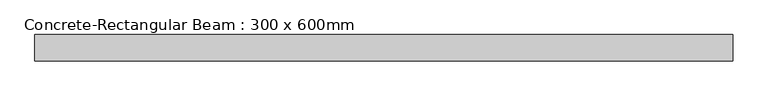
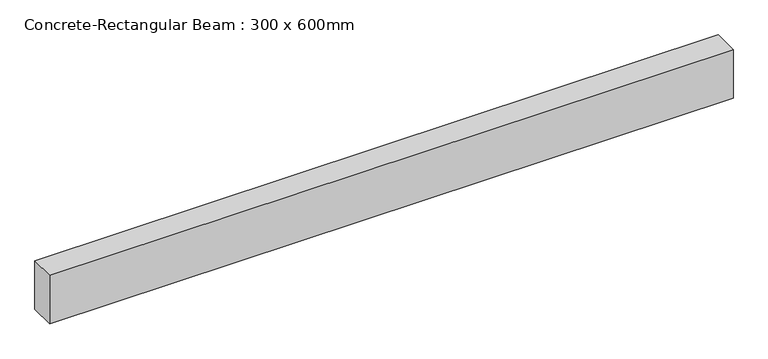
"""IFC4 building model written with IfcOpenShell, lengths in millimetres: beam geometry, Concrete-Rectangular Beam : 300 x 600mm."""

from ifc_helpers import new_model, si_unit, frame, origin, place, context, project, spatial, polyline, outline, extrude, source, transform, mapped, element, save


def concrete_rectangular_beam_300_x_600mm_0e8e550c(model_context):
    return source(origin(), model_context, "Body", "SweptSolid", [
        extrude(outline(polyline([(4000.0, 150.0), (4000.0, -150.0), (-4000.0, -150.0), (-4000.0, 150.0), (4000.0, 150.0)])), frame((0.0, 0.0, -300.0), z_axis=(0.0, 0.0, 1.0), x_axis=(1.0, 0.0, 0.0)), (0.0, 0.0, 1.0), 600.0),
    ])


if __name__ == "__main__":
    model = new_model("IFC4")
    model_context = context("Model", 3, world=origin())
    ifc_project = project(units=[si_unit("LENGTHUNIT", "METRE", prefix="MILLI")], contexts=[model_context])
    site = spatial("IfcSite", under=ifc_project)
    building = spatial("IfcBuilding", under=site)
    placement = place(None, origin())
    concrete_rectangular_beam_300_x_600mm_shape = concrete_rectangular_beam_300_x_600mm_0e8e550c(model_context)
    element("IfcBeam", 1, ObjectType="Concrete-Rectangular Beam : 300 x 600mm", at=placement, inside=building, context=model_context, shape_type="MappedRepresentation", body=[
        mapped(concrete_rectangular_beam_300_x_600mm_shape, transform((0.0, 0.0, 0.0), x_axis=(1.0, 0.0, 0.0), y_axis=(0.0, 1.0, 0.0), z_axis=(0.0, 0.0, 1.0))),
    ])
    save(model, "model.ifc")

# Revit data of these elements
# Type "Concrete-Rectangular Beam : 300 x 600mm"
#   Length [instance default] = 1524 mm
#   b = 300 mm
#   h = 600 mm
#   Structural Material [instance default] = Concrete, Cast-in-Place gray
#   Assembly Code = ""
# Element 1 (IfcBeam, "Concrete-Rectangular Beam : 300 x 600mm")
#   Materials on its faces: "Concrete, Cast-in-Place gray"
# Materials
#   "Concrete, Cast-in-Place gray": class "Concrete", colour RGB 192 192 192, transparency 0, Description = "Cast-in-place concrete", Cost = 0
